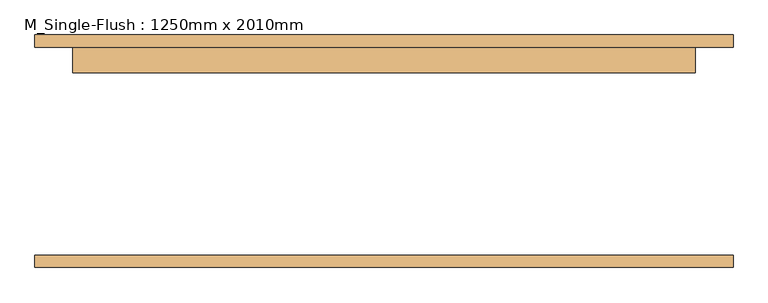
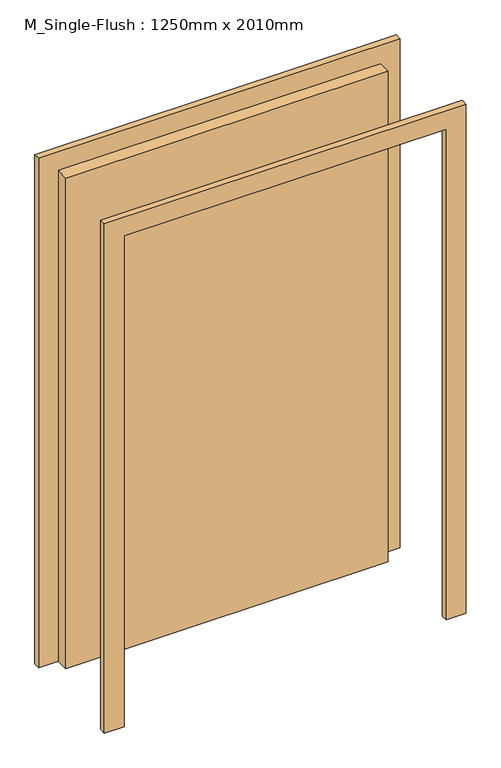
"""IFC4 building model written with IfcOpenShell, lengths in millimetres: door geometry, M_Single-Flush : 1250mm x 2010mm."""

from ifc_helpers import new_model, si_unit, frame, origin, origin_with_axes, place, context, project, spatial, polyline, outline, extrude, source, transform, mapped, element, save


def m_single_flush_1250mm_x_2010mm_0100e384(model_context):
    return source(origin(), model_context, "Body", "SweptSolid", [
        extrude(outline(polyline([(2086.0, -701.0), (0.0, -701.0), (0.0, -625.0), (2010.0, -625.0), (2010.0, 625.0), (0.0, 625.0), (0.0, 701.0), (2086.0, 701.0), (2086.0, -701.0)])), frame((0.0, 208.5, 0.0), z_axis=(0.0, 1.0, 0.0), x_axis=(0.0, 0.0, 1.0)), (0.0, 0.0, 1.0), 25.0),
        extrude(outline(polyline([(2086.0, 701.0), (2086.0, -701.0), (0.0, -701.0), (0.0, -625.0), (2010.0, -625.0), (2010.0, 625.0), (0.0, 625.0), (0.0, 701.0), (2086.0, 701.0)])), frame((0.0, -233.5, 0.0), z_axis=(0.0, 1.0, 0.0), x_axis=(0.0, 0.0, 1.0)), (0.0, 0.0, 1.0), 25.0),
        extrude(outline(polyline([(625.0, 157.5), (-625.0, 157.5), (-625.0, 208.5), (625.0, 208.5), (625.0, 157.5)])), origin_with_axes(), (0.0, 0.0, 1.0), 2010.0),
    ])


if __name__ == "__main__":
    model = new_model("IFC4")
    model_context = context("Model", 3, world=origin())
    ifc_project = project(units=[si_unit("LENGTHUNIT", "METRE", prefix="MILLI")], contexts=[model_context])
    site = spatial("IfcSite", under=ifc_project)
    building = spatial("IfcBuilding", under=site)
    placement = place(None, origin())
    m_single_flush_1250mm_x_2010mm_shape = m_single_flush_1250mm_x_2010mm_0100e384(model_context)
    element("IfcDoor", 1, ObjectType="M_Single-Flush : 1250mm x 2010mm", at=placement, inside=building, context=model_context, shape_type="MappedRepresentation", body=[
        mapped(m_single_flush_1250mm_x_2010mm_shape, transform((0.0, 0.0, 0.0), x_axis=(1.0, 0.0, 0.0), y_axis=(0.0, 1.0, 0.0), z_axis=(0.0, 0.0, 1.0))),
    ])
    save(model, "model.ifc")

# Revit data of these elements
# Type "M_Single-Flush : 1250mm x 2010mm"
#   Manufacturer = "Manufacturer"
#   Type Mark = "33"
#   Construction Type = "Construction Type"
#   Fire Rating = "Fire Rating"
#   AccessibilityPerformance = "AccessibilityPerformance"
#   CodePerformance = "CodePerformance"
#   IsFireExit = "IsFireExit"
#   ConstructionType = "ConstructionType"
#   GlazingAreaFraction = "GlazingAreaFraction"
#   OperationType = "OperationType"
#   Area = "Area"
#   Color = "Color"
#   Constituents = "Constituents"
#   Features = "Features"
#   Finish = "Finish"
#   Grade = "Grade"
#   Material = "Material"
#   ModelReference = "ModelReference"
#   NominalHeight = "NominalHeight"
#   NominalLength = "NominalLength"
#   NominalWidth = "NominalWidth"
#   ProductionYear = "ProductionYear"
#   Reference = "Reference"
#   Shape = "Shape"
#   Size = "Size"
#   SustainabilityPerformance = "SustainabilityPerformance"
#   WarrantyDescription = "WarrantyDescription"
#   WarrantyDurationLabor = "WarrantyDurationLabor"
#   WarrantyDurationParts = "WarrantyDurationParts"
#   WarrantyGuarantorLabor = "WarrantyGuarantorLabor"
#   WarrantyGuarantorParts = "WarrantyGuarantorParts"
#   ExpectedLife = "ExpectedLife"
#   ReplacementCost = "ReplacementCost"
#   AssetAccountingType = "FIXED"
#   ModelLabel = "ModelLabel"
#   Thickness = 0.051 m
#   Height = 2.010 m
#   Trim Projection Ext = 0.025 m
#   Trim Projection Int = 0.025 m
#   Trim Width = 0.076 m
#   Width = 1.250 m
#   Function = 1
#   Door Material = Door - Panel
#   Frame Material = Door - Frame
#   Wall Closure = (empty or 0)
# Element 1 (IfcDoor, "M_Single-Flush : 1250mm x 2010mm")
#   Materials on its faces: "Door - Frame", "Door - Panel"
# Materials
#   "Door - Panel": class "Wood", colour RGB 210 159 95, transparency 0
#   "Door - Frame": class "Miscellaneous", colour RGB 118 70 51, transparency 0
